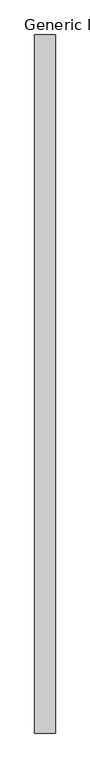
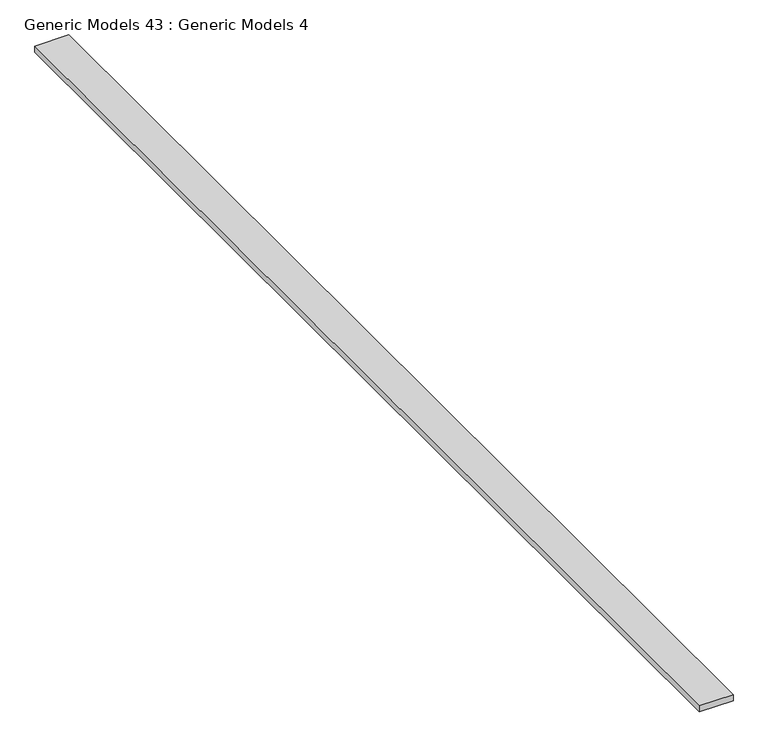
"""IFC4 building model written with IfcOpenShell, lengths in millimetres: proxy geometry, Generic Models 43 : Generic Models 4."""

from ifc_helpers import new_model, si_unit, frame, origin, place, context, project, spatial, polyline, outline, extrude, source, transform, mapped, element, save


def generic_models_43_generic_models_4_1fbcf8ac(model_context):
    return source(origin(), model_context, "Body", "SweptSolid", [
        extrude(outline(polyline([(-9277.5236296, 7054.2769662), (-9417.2236296, 7054.2769662), (-9417.2236296, 11778.6769662), (-9277.5236296, 11778.6769662), (-9277.5236296, 7054.2769662)])), frame((0.0, 0.0, 126383.796), z_axis=(0.0, 0.0, 1.0), x_axis=(1.0, 0.0, 0.0)), (0.0, 0.0, 1.0), 25.4),
    ])


if __name__ == "__main__":
    model = new_model("IFC4")
    model_context = context("Model", 3, world=origin())
    ifc_project = project(units=[si_unit("LENGTHUNIT", "METRE", prefix="MILLI")], contexts=[model_context])
    site = spatial("IfcSite", under=ifc_project)
    building = spatial("IfcBuilding", under=site)
    placement = place(None, origin())
    generic_models_43_generic_models_4_shape = generic_models_43_generic_models_4_1fbcf8ac(model_context)
    element("IfcBuildingElementProxy", 1, Name="Generic Models 43 : Generic Models 4", ObjectType="Generic Models 43 : Generic Models 4", at=placement, inside=building, context=model_context, shape_type="MappedRepresentation", body=[
        mapped(generic_models_43_generic_models_4_shape, transform((0.0, 0.0, 0.0), x_axis=(1.0, 0.0, 0.0), y_axis=(0.0, 1.0, 0.0), z_axis=(0.0, 0.0, 1.0))),
    ])
    save(model, "model.ifc")

# Revit data of these elements
# Element 1 (IfcBuildingElementProxy, "Generic Models 43 : Generic Models 4")
#   Materials on its faces: "_2X BLOCKING AS REQUIRED"
# Materials
#   "_2X BLOCKING AS REQUIRED": class "Generic", colour RGB 177 130 114, transparency 0, Cost = 0
